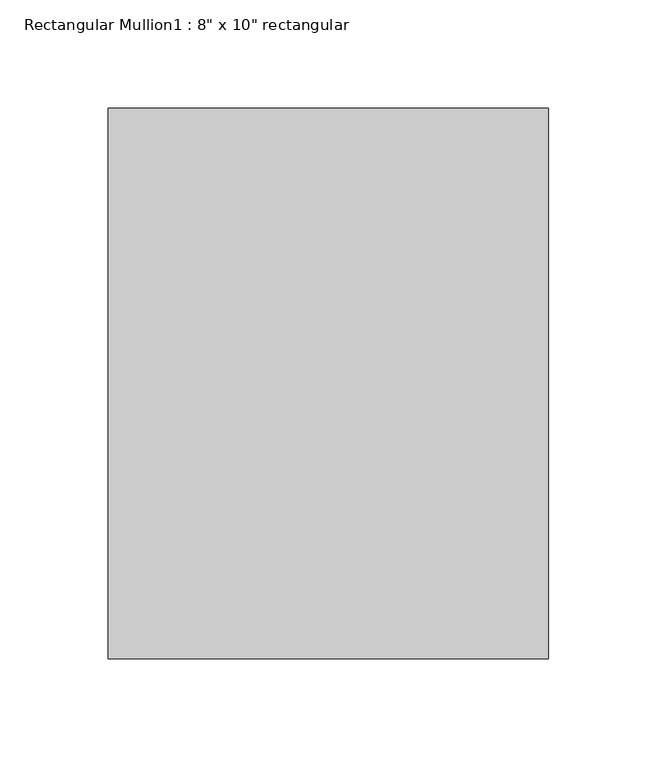
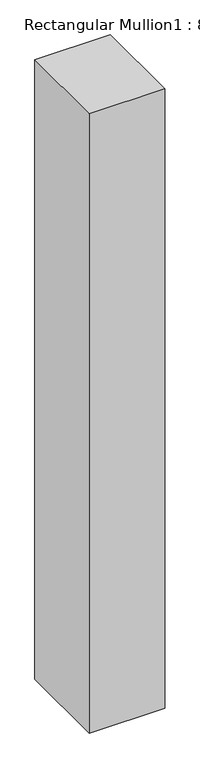
"""IFC4 building model written with IfcOpenShell, lengths in millimetres: member geometry."""

from ifc_helpers import new_model, si_unit, frame, origin, place, context, project, spatial, polyline, outline, extrude, source, transform, mapped, element, save


def member_136c1585(model_context):
    return source(origin(), model_context, "Body", "SweptSolid", [
        extrude(outline(polyline([(0.0, 127.0), (0.0, -127.0), (-203.2, -127.0), (-203.2, 127.0), (0.0, 127.0)])), frame((0.0, 0.0, -1765.3), z_axis=(0.0, 0.0, 1.0), x_axis=(1.0, 0.0, 0.0)), (0.0, 0.0, 1.0), 1765.3),
    ])


if __name__ == "__main__":
    model = new_model("IFC4")
    model_context = context("Model", 3, world=origin())
    ifc_project = project(units=[si_unit("LENGTHUNIT", "METRE", prefix="MILLI")], contexts=[model_context])
    site = spatial("IfcSite", under=ifc_project)
    building = spatial("IfcBuilding", under=site)
    placement = place(None, origin())
    member_shape = member_136c1585(model_context)
    element("IfcMember", 1, ObjectType="Rectangular Mullion1 : 8\" x 10\" rectangular", at=placement, inside=building, context=model_context, shape_type="MappedRepresentation", body=[
        mapped(member_shape, transform((0.0, 0.0, 0.0), x_axis=(1.0, 0.0, 0.0), y_axis=(0.0, 1.0, 0.0), z_axis=(0.0, 0.0, 1.0))),
    ])
    save(model, "model.ifc")

# Revit data of these elements
# Type "Rectangular Mullion1 : 8\" x 10\" rectangular"
#   built-in parameter 1007304 = 0.833333 (stored number, unit not read)
#   built-in parameter 1007301 = 0.333333 (stored number, unit not read)
#   built-in parameter 1007300 = 0.333333 (stored number, unit not read)
# Element 1 (IfcMember, "Rectangular Mullion1 : 8\" x 10\" rectangular")
#   Materials on its faces: "support-frame"
# Materials
#   "support-frame": class "Unassigned", colour RGB 233 233 233, transparency 0, Cost = 0
